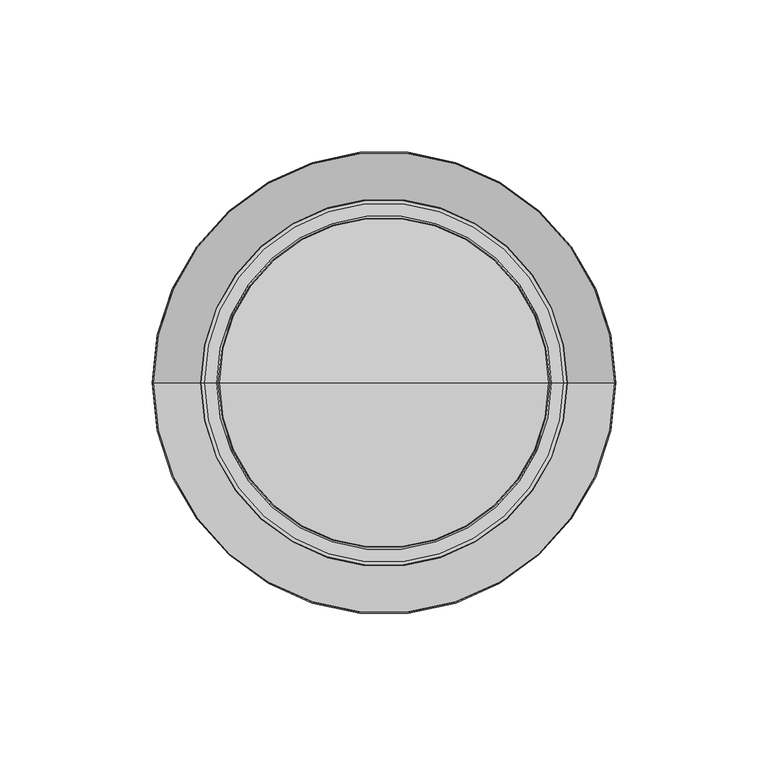
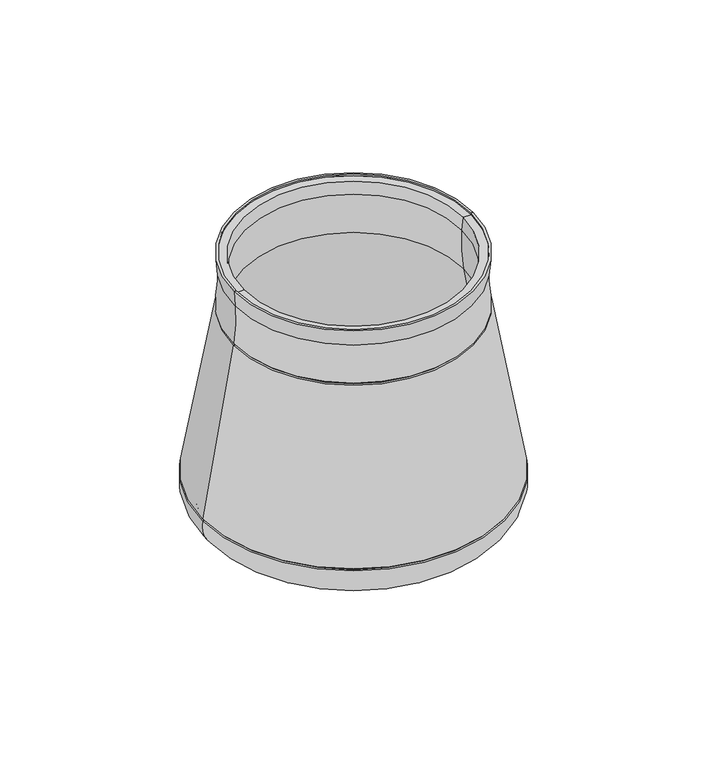
"""IFC4 building model written with IfcOpenShell, lengths in millimetres: proxy geometry, Smoothie_Maker_ : Smoothie_Maker_."""

from ifc_helpers import new_model, si_unit, point, frame, origin, place, context, project, spatial, polyline, circle_curve, ellipse_curve, trimmed, source, transform, mapped, element, save
from ifc_brep_helpers import plane_surface, cylinder_surface, revolved_surface, advanced_brep


def generic_models_cb25b0b2(model_context):
    return source(origin(), model_context, "Body", "AdvancedBrep", [
        advanced_brep(
        [(60.0, 0.0, 150.0), (-60.0, 0.0, 150.0), (-59.0, 0.0, 150.0), (59.0, 0.0, 150.0), (75.5984681, 0.0, 34.8567262), (-75.5984681, 0.0, 34.8567262), (-60.330808, 0.0, 121.4439292), (60.330808, 0.0, 121.4439292), (74.5830415, 0.0, 34.8567262), (-74.5830415, 0.0, 34.8567262), (74.7566897, 0.0, 33.8719184), (-74.7566897, 0.0, 33.8719184), (75.7721163, 0.0, 33.8719184), (-75.7721163, 0.0, 33.8719184), (64.1625838, 0.0, 16.6043835), (-64.1625838, 0.0, 16.6043835), (0.0, 0.0, 9.76351), (59.3004602, 0.0, 142.0042232), (-59.3004602, 0.0, 142.0042232), (60.1544811, 0.0, 122.4439292), (-60.1544811, 0.0, 122.4439292), (59.1544811, 0.0, 122.4439292), (-59.1544811, 0.0, 122.4439292), (59.1544811, 0.0, 121.4439292), (-59.1544811, 0.0, 121.4439292), (63.1083892, 0.0, 21.4919876), (-63.1083892, 0.0, 21.4919876), (0.0, 0.0, 14.76351), (70.8480775, 0.0, 33.0036775), (-70.8480775, 0.0, 33.0036775), (55.2304423, 0.0, 121.5756883), (-55.2304423, 0.0, 121.5756883), (54.3194867, 0.0, 142.440002), (-54.3194867, 0.0, 142.440002), (54.8934121, 0.0, 149.0), (-54.8934121, 0.0, 149.0), (59.0, 0.0, 149.0), (-59.0, 0.0, 149.0)],
        [
            (0, 1, circle_curve(frame((0.0, 0.0, 150.0), z_axis=(0.0, 0.0, 1.0), x_axis=(-1.0, 0.0, 0.0)), 60.0)),
            (1, 2),
            (2, 3, circle_curve(frame((0.0, 0.0, 150.0), z_axis=(0.0, 0.0, -1.0), x_axis=(-1.0, 0.0, 0.0)), 59.0)),
            (3, 0),
            (1, 0, circle_curve(frame((0.0, 0.0, 150.0), z_axis=(0.0, 0.0, 1.0), x_axis=(-1.0, 0.0, 0.0)), 60.0)),
            (3, 2, circle_curve(frame((0.0, 0.0, 150.0), z_axis=(0.0, 0.0, -1.0), x_axis=(-1.0, 0.0, 0.0)), 59.0)),
            (4, 5, circle_curve(frame((0.0, 0.0, 34.8567262), z_axis=(0.0, 0.0, 1.0), x_axis=(-1.0, 0.0, 0.0)), 75.5984681)),
            (5, 6),
            (6, 7, circle_curve(frame((0.0, 0.0, 121.4439292), z_axis=(0.0, 0.0, -1.0), x_axis=(-1.0, 0.0, 0.0)), 60.330808)),
            (7, 4),
            (5, 4, circle_curve(frame((0.0, 0.0, 34.8567262), z_axis=(0.0, 0.0, 1.0), x_axis=(-1.0, 0.0, 0.0)), 75.5984681)),
            (7, 6, circle_curve(frame((0.0, 0.0, 121.4439292), z_axis=(0.0, 0.0, -1.0), x_axis=(-1.0, 0.0, 0.0)), 60.330808)),
            (8, 9, circle_curve(frame((0.0, 0.0, 34.8567262), z_axis=(0.0, 0.0, 1.0), x_axis=(-1.0, 0.0, 0.0)), 74.5830415)),
            (9, 5),
            (4, 8),
            (9, 8, circle_curve(frame((0.0, 0.0, 34.8567262), z_axis=(0.0, 0.0, 1.0), x_axis=(-1.0, 0.0, 0.0)), 74.5830415)),
            (10, 11, circle_curve(frame((0.0, 0.0, 33.8719184), z_axis=(0.0, 0.0, 1.0), x_axis=(-1.0, 0.0, 0.0)), 74.7566897)),
            (11, 9),
            (8, 10),
            (11, 10, circle_curve(frame((0.0, 0.0, 33.8719184), z_axis=(0.0, 0.0, 1.0), x_axis=(-1.0, 0.0, 0.0)), 74.7566897)),
            (12, 13, circle_curve(frame((0.0, 0.0, 33.8719184), z_axis=(0.0, 0.0, 1.0), x_axis=(-1.0, 0.0, 0.0)), 75.7721163)),
            (13, 11),
            (10, 12),
            (13, 12, circle_curve(frame((0.0, 0.0, 33.8719184), z_axis=(0.0, 0.0, 1.0), x_axis=(-1.0, 0.0, 0.0)), 75.7721163)),
            (14, 15, circle_curve(frame((0.0, 0.0, 16.6043835), z_axis=(0.0, 0.0, 1.0), x_axis=(-1.0, 0.0, 0.0)), 64.1625838)),
            (15, 13, circle_curve(frame((-61.0, 0.0, 31.2671958), z_axis=(0.0, 1.0, 0.0), x_axis=(1.0, 0.0, 0.0)), 15.0)),
            (12, 14, circle_curve(frame((61.0, 0.0, 31.2671958), z_axis=(0.0, 1.0, 0.0), x_axis=(-1.0, 0.0, 0.0)), 15.0)),
            (15, 14, circle_curve(frame((0.0, 0.0, 16.6043835), z_axis=(0.0, 0.0, 1.0), x_axis=(-1.0, 0.0, 0.0)), 64.1625838)),
            (16, 15, circle_curve(frame((0.0, 0.0, 314.0839102), z_axis=(0.0, 1.0, 0.0), x_axis=(1.0, 0.0, 0.0)), 304.3204002)),
            (14, 16, circle_curve(frame((0.0, 0.0, 314.0839102), z_axis=(0.0, 1.0, 0.0), x_axis=(-1.0, 0.0, 0.0)), 304.3204002)),
            (17, 18, circle_curve(frame((0.0, 0.0, 142.0042232), z_axis=(0.0, 0.0, 1.0), x_axis=(-1.0, 0.0, 0.0)), 59.3004602)),
            (18, 1),
            (0, 17),
            (18, 17, circle_curve(frame((0.0, 0.0, 142.0042232), z_axis=(0.0, 0.0, 1.0), x_axis=(-1.0, 0.0, 0.0)), 59.3004602)),
            (19, 20, circle_curve(frame((0.0, 0.0, 122.4439292), z_axis=(0.0, 0.0, 1.0), x_axis=(-1.0, 0.0, 0.0)), 60.1544811)),
            (20, 18, circle_curve(frame((-134.0150625, 0.0, 135.4675425), z_axis=(0.0, -1.0, 0.0), x_axis=(1.0, 0.0, 0.0)), 75.0)),
            (17, 19, circle_curve(frame((134.0150625, 0.0, 135.4675425), z_axis=(0.0, -1.0, 0.0), x_axis=(-1.0, 0.0, 0.0)), 75.0)),
            (20, 19, circle_curve(frame((0.0, 0.0, 122.4439292), z_axis=(0.0, 0.0, 1.0), x_axis=(-1.0, 0.0, 0.0)), 60.1544811)),
            (21, 22, circle_curve(frame((0.0, 0.0, 122.4439292), z_axis=(0.0, 0.0, 1.0), x_axis=(-1.0, 0.0, 0.0)), 59.1544811)),
            (22, 20),
            (19, 21),
            (22, 21, circle_curve(frame((0.0, 0.0, 122.4439292), z_axis=(0.0, 0.0, 1.0), x_axis=(-1.0, 0.0, 0.0)), 59.1544811)),
            (23, 24, circle_curve(frame((0.0, 0.0, 121.4439292), z_axis=(0.0, 0.0, 1.0), x_axis=(-1.0, 0.0, 0.0)), 59.1544811)),
            (24, 22),
            (21, 23),
            (24, 23, circle_curve(frame((0.0, 0.0, 121.4439292), z_axis=(0.0, 0.0, 1.0), x_axis=(-1.0, 0.0, 0.0)), 59.1544811)),
            (6, 24),
            (23, 7),
            (25, 26, circle_curve(frame((0.0, 0.0, 21.4919876), z_axis=(0.0, 0.0, 1.0), x_axis=(-1.0, 0.0, 0.0)), 63.1083892)),
            (26, 27, circle_curve(frame((0.0, 0.0, 314.0839102), z_axis=(0.0, -1.0, 0.0), x_axis=(1.0, 0.0, 0.0)), 299.3204002)),
            (27, 25, circle_curve(frame((0.0, 0.0, 314.0839102), z_axis=(0.0, -1.0, 0.0), x_axis=(-1.0, 0.0, 0.0)), 299.3204002)),
            (26, 25, circle_curve(frame((0.0, 0.0, 21.4919876), z_axis=(0.0, 0.0, 1.0), x_axis=(-1.0, 0.0, 0.0)), 63.1083892)),
            (28, 29, circle_curve(frame((0.0, 0.0, 33.0036775), z_axis=(0.0, 0.0, 1.0), x_axis=(-1.0, 0.0, 0.0)), 70.8480775)),
            (29, 26, circle_curve(frame((-61.0, 0.0, 31.2671958), z_axis=(0.0, -1.0, 0.0), x_axis=(1.0, 0.0, 0.0)), 10.0)),
            (25, 28, circle_curve(frame((61.0, 0.0, 31.2671958), z_axis=(0.0, -1.0, 0.0), x_axis=(-1.0, 0.0, 0.0)), 10.0)),
            (29, 28, circle_curve(frame((0.0, 0.0, 33.0036775), z_axis=(0.0, 0.0, 1.0), x_axis=(-1.0, 0.0, 0.0)), 70.8480775)),
            (30, 31, circle_curve(frame((0.0, 0.0, 121.5756883), z_axis=(0.0, 0.0, 1.0), x_axis=(-1.0, 0.0, 0.0)), 55.2304423)),
            (31, 29),
            (28, 30),
            (31, 30, circle_curve(frame((0.0, 0.0, 121.5756883), z_axis=(0.0, 0.0, 1.0), x_axis=(-1.0, 0.0, 0.0)), 55.2304423)),
            (32, 33, circle_curve(frame((0.0, 0.0, 142.440002), z_axis=(0.0, 0.0, 1.0), x_axis=(-1.0, 0.0, 0.0)), 54.3194867)),
            (33, 31, circle_curve(frame((-134.0150625, 0.0, 135.4675425), z_axis=(0.0, 1.0, 0.0), x_axis=(1.0, 0.0, 0.0)), 80.0)),
            (30, 32, circle_curve(frame((134.0150625, 0.0, 135.4675425), z_axis=(0.0, 1.0, 0.0), x_axis=(-1.0, 0.0, 0.0)), 80.0)),
            (33, 32, circle_curve(frame((0.0, 0.0, 142.440002), z_axis=(0.0, 0.0, 1.0), x_axis=(-1.0, 0.0, 0.0)), 54.3194867)),
            (34, 35, circle_curve(frame((0.0, 0.0, 149.0), z_axis=(0.0, 0.0, 1.0), x_axis=(-1.0, 0.0, 0.0)), 54.8934121)),
            (35, 33),
            (32, 34),
            (35, 34, circle_curve(frame((0.0, 0.0, 149.0), z_axis=(0.0, 0.0, 1.0), x_axis=(-1.0, 0.0, 0.0)), 54.8934121)),
            (36, 37, circle_curve(frame((0.0, 0.0, 149.0), z_axis=(0.0, 0.0, 1.0), x_axis=(-1.0, 0.0, 0.0)), 59.0)),
            (37, 35),
            (34, 36),
            (37, 36, circle_curve(frame((0.0, 0.0, 149.0), z_axis=(0.0, 0.0, 1.0), x_axis=(-1.0, 0.0, 0.0)), 59.0)),
            (2, 37),
            (36, 3),
        ],
        [
            plane_surface(frame((0.0, 0.0, 150.0), z_axis=(0.0, 0.0, 1.0), x_axis=(-1.0, 0.0, 0.0))),
            revolved_surface(polyline([(-60.330808, 0.0, 121.4439292), (-75.5984681, 0.0, 34.8567262)]), (0.0, 0.0, 14.76351), (0.0, 0.0, -1.0)),
            plane_surface(frame((0.0, 0.0, 34.8567262), z_axis=(0.0, 0.0, -1.0), x_axis=(-1.0, 0.0, 0.0))),
            revolved_surface(polyline([(-74.5830415, 0.0, 34.8567262), (-74.7566897, 0.0, 33.8719184)]), (0.0, 0.0, 14.76351), (0.0, 0.0, -1.0)),
            plane_surface(frame((0.0, 0.0, 33.8719184), z_axis=(0.0, 0.0, 1.0), x_axis=(-1.0, 0.0, 0.0))),
            revolved_surface(trimmed(ellipse_curve(frame((-61.0, 0.0, 31.2671958), z_axis=(0.0, -1.0, 0.0), x_axis=(1.0, 0.0, 0.0)), 15.0, 15.0), [point((-75.7721163, 0.0, 33.8719184))], [point((-64.1625838, 0.0, 16.6043835))], True, "CARTESIAN"), (0.0, 0.0, 14.76351), (0.0, 0.0, -1.0)),
            revolved_surface(trimmed(ellipse_curve(frame((0.0, 0.0, 314.0839102), z_axis=(0.0, -1.0, 0.0), x_axis=(1.0, 0.0, 0.0)), 304.3204002, 304.3204002), [point((-64.1625838, 0.0, 16.6043835))], [point((0.0, 0.0, 9.76351))], True, "CARTESIAN"), (0.0, 0.0, 14.76351), (0.0, 0.0, -1.0)),
            revolved_surface(polyline([(-60.0, 0.0, 150.0), (-59.3004602, 0.0, 142.0042232)]), (0.0, 0.0, 14.76351), (0.0, 0.0, -1.0)),
            revolved_surface(trimmed(ellipse_curve(frame((-134.0150625, 0.0, 135.4675425), z_axis=(0.0, 1.0, 0.0), x_axis=(1.0, 0.0, 0.0)), 75.0, 75.0), [point((-59.3004602, 0.0, 142.0042232))], [point((-60.1544811, 0.0, 122.4439292))], True, "CARTESIAN"), (0.0, 0.0, 14.76351), (0.0, 0.0, -1.0)),
            plane_surface(frame((0.0, 0.0, 122.4439292), z_axis=(0.0, 0.0, -1.0), x_axis=(-1.0, 0.0, 0.0))),
            cylinder_surface(frame((0.0, 0.0, 14.76351), z_axis=(0.0, 0.0, -1.0), x_axis=(-1.0, 0.0, 0.0)), 59.1544811),
            plane_surface(frame((0.0, 0.0, 121.4439292), z_axis=(0.0, 0.0, 1.0), x_axis=(-1.0, 0.0, 0.0))),
            revolved_surface(trimmed(ellipse_curve(frame((0.0, 0.0, 314.0839102), z_axis=(0.0, 1.0, 0.0), x_axis=(1.0, 0.0, 0.0)), 299.3204002, 299.3204002), [point((0.0, 0.0, 14.76351))], [point((-63.1083892, 0.0, 21.4919876))], True, "CARTESIAN"), (0.0, 0.0, 14.76351), (0.0, 0.0, -1.0)),
            revolved_surface(trimmed(ellipse_curve(frame((-61.0, 0.0, 31.2671958), z_axis=(0.0, 1.0, 0.0), x_axis=(1.0, 0.0, 0.0)), 10.0, 10.0), [point((-63.1083892, 0.0, 21.4919876))], [point((-70.8480775, 0.0, 33.0036775))], True, "CARTESIAN"), (0.0, 0.0, 14.76351), (0.0, 0.0, -1.0)),
            revolved_surface(polyline([(-70.8480775, 0.0, 33.0036775), (-55.2304423, 0.0, 121.5756883)]), (0.0, 0.0, 14.76351), (0.0, 0.0, -1.0)),
            revolved_surface(trimmed(ellipse_curve(frame((-134.0150625, 0.0, 135.4675425), z_axis=(0.0, -1.0, 0.0), x_axis=(1.0, 0.0, 0.0)), 80.0, 80.0), [point((-55.2304423, 0.0, 121.5756883))], [point((-54.3194867, 0.0, 142.440002))], True, "CARTESIAN"), (0.0, 0.0, 14.76351), (0.0, 0.0, -1.0)),
            revolved_surface(polyline([(-54.3194867, 0.0, 142.440002), (-54.8934121, 0.0, 149.0)]), (0.0, 0.0, 14.76351), (0.0, 0.0, -1.0)),
            plane_surface(frame((0.0, 0.0, 149.0), z_axis=(0.0, 0.0, 1.0), x_axis=(-1.0, 0.0, 0.0))),
            revolved_surface(polyline([(-59.0, 0.0, 149.0), (-59.0, 0.0, 150.0)]), (0.0, 0.0, 14.76351), (0.0, 0.0, -1.0)),
        ],
        [
            (0, [[1, 2, 3, 4]]),
            (0, [[5, -4, 6, -2]]),
            (1, [[7, 8, 9, 10]]),
            (1, [[11, -10, 12, -8]]),
            (2, [[13, 14, -7, 15]]),
            (2, [[16, -15, -11, -14]]),
            (3, [[17, 18, -13, 19]]),
            (3, [[20, -19, -16, -18]]),
            (4, [[21, 22, -17, 23]]),
            (4, [[24, -23, -20, -22]]),
            (5, [[25, 26, -21, 27]]),
            (5, [[28, -27, -24, -26]]),
            (6, [[29, -25, 30]]),
            (6, [[-30, -28, -29]]),
            (7, [[31, 32, -1, 33]]),
            (7, [[34, -33, -5, -32]]),
            (8, [[35, 36, -31, 37]]),
            (8, [[38, -37, -34, -36]]),
            (9, [[39, 40, -35, 41]]),
            (9, [[42, -41, -38, -40]]),
            (10, [[43, 44, -39, 45]]),
            (10, [[46, -45, -42, -44]]),
            (11, [[-9, 47, -43, 48]]),
            (11, [[-12, -48, -46, -47]]),
            (12, [[49, 50, 51]]),
            (12, [[52, -51, -50]]),
            (13, [[53, 54, -49, 55]]),
            (13, [[56, -55, -52, -54]]),
            (14, [[57, 58, -53, 59]]),
            (14, [[60, -59, -56, -58]]),
            (15, [[61, 62, -57, 63]]),
            (15, [[64, -63, -60, -62]]),
            (16, [[65, 66, -61, 67]]),
            (16, [[68, -67, -64, -66]]),
            (17, [[69, 70, -65, 71]]),
            (17, [[72, -71, -68, -70]]),
            (18, [[-3, 73, -69, 74]]),
            (18, [[-6, -74, -72, -73]]),
        ],
    ),
    ])


if __name__ == "__main__":
    model = new_model("IFC4")
    model_context = context("Model", 3, world=origin())
    ifc_project = project(units=[si_unit("LENGTHUNIT", "METRE", prefix="MILLI")], contexts=[model_context])
    site = spatial("IfcSite", under=ifc_project)
    building = spatial("IfcBuilding", under=site)
    placement = place(None, origin())
    generic_models_shape = generic_models_cb25b0b2(model_context)
    element("IfcBuildingElementProxy", 1, Name="Smoothie_Maker_ : Smoothie_Maker_", ObjectType="Smoothie_Maker_ : Smoothie_Maker_", at=placement, inside=building, context=model_context, shape_type="MappedRepresentation", body=[
        mapped(generic_models_shape, transform((0.0, 0.0, 0.0), x_axis=(1.0, 0.0, 0.0), y_axis=(0.0, 1.0, 0.0), z_axis=(0.0, 0.0, 1.0))),
    ])
    save(model, "model.ifc")

# Revit data of these elements
# Type "Smoothie_Maker_ : Smoothie_Maker_"
#   Smoothie Maker - Silver Plastic = Smoothie Maker - Silver Plastic
#   Smoothie Maker - Drink Container = Smoothie Maker - Drink Container
#   Smoothie Maker - Dials = Smoothie Maker - Dials
#   Smoothie Maker - Blades = Smoothie Maker - Blades
#   Smoothie Maker - Black Plastic = Smoothie Maker - Black Plastic
#   Default Elevation = 0
# Element 1 (IfcBuildingElementProxy, "Smoothie_Maker_ : Smoothie_Maker_")
#   Materials on its faces: "Smoothie Maker - Drink Container", "Smoothie Maker - Silver Plastic", "Smoothie Maker - Blades", "Smoothie Maker - Dials"
# Materials
#   "Smoothie Maker - Silver Plastic": class "Generic", colour RGB 120 120 120, transparency 0, Cost = 0
#   "Smoothie Maker - Drink Container": class "Generic", colour RGB 120 120 120, transparency 0, Cost = 0
#   "Smoothie Maker - Dials": class "Generic", colour RGB 120 120 120, transparency 0, Cost = 0
#   "Smoothie Maker - Blades": class "Generic", colour RGB 120 120 120, transparency 0, Cost = 0
#   "Smoothie Maker - Black Plastic": class "Generic", colour RGB 120 120 120, transparency 0, Cost = 0
